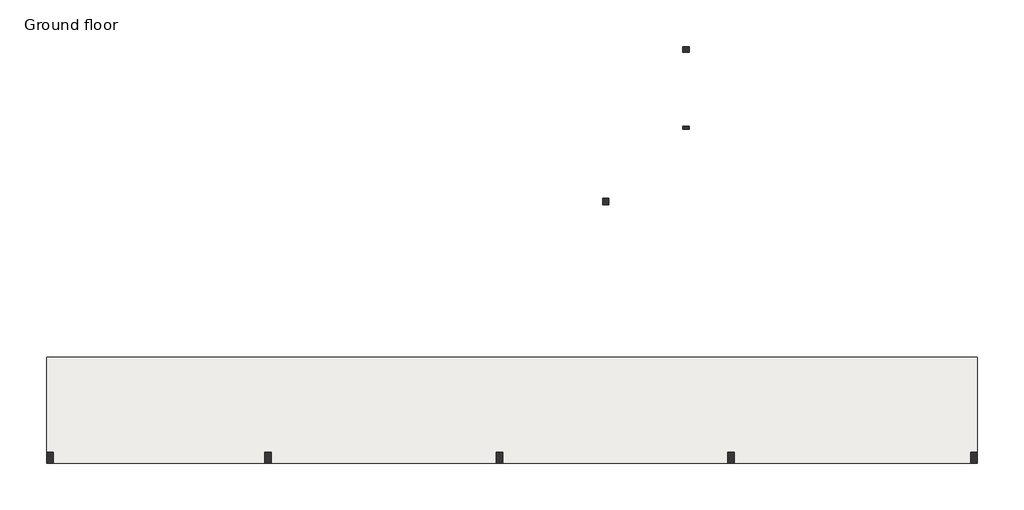
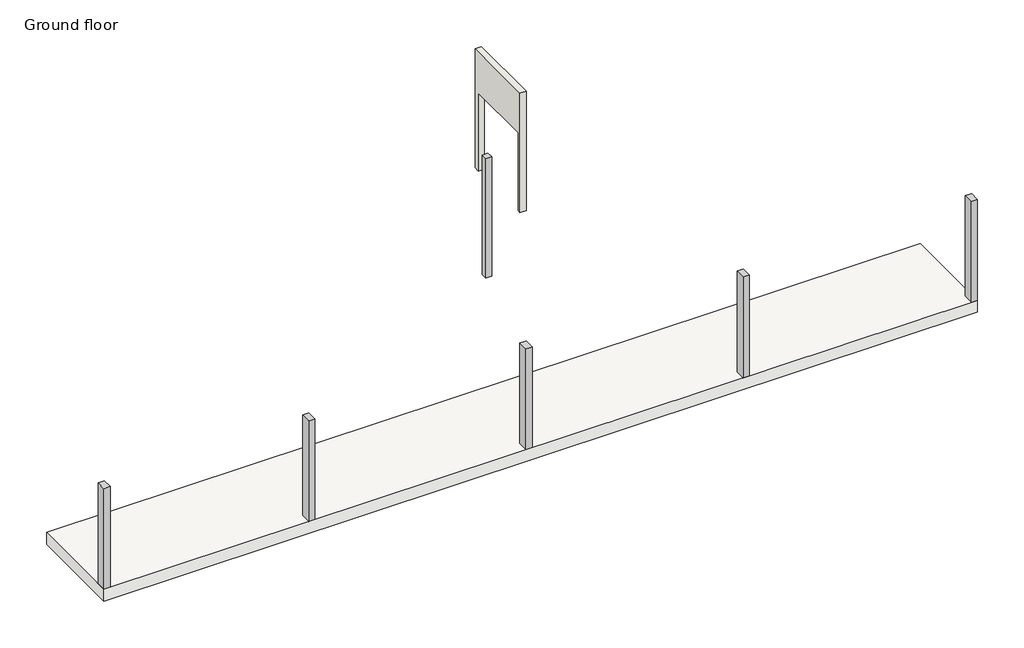
# One storey: 6 columns, 1 slab, 1 wall.
"""IFC4 building model written with IfcOpenShell, lengths in millimetres."""

import ifcopenshell
import ifcopenshell.guid

model = None  # the IFC model being written
_history = None  # IfcOwnerHistory: only IFC2X3 demands one
_inside = {}  # id of a spatial element -> (the spatial element, [elements in it])
_under = {}  # id of a project, library or spatial element -> (it, [spatial elements below it])
_declared = {}  # id of a project -> (the project, [libraries it declares])
_typed = {}  # id of a type object -> (the type object, [elements of that type])
_made_of = {}  # id of a material, layer set ... -> (it, [elements and type objects made of it])


def new_model(schema):
    """Start an empty IFC model of exactly this schema.

    Asked for "IFC4X3", IfcOpenShell would pick the latest addendum, in which some entities
    have other attributes; the version numbers below select the first issue.
    IFC2X3 requires an IfcOwnerHistory on every rooted entity: one is made here for all.
    """
    global model, _history
    if schema == "IFC4X3":
        model = ifcopenshell.file(schema_version=(4, 3, 0, 0))
    else:
        model = ifcopenshell.file(schema=schema)
    _inside.clear()
    _under.clear()
    _declared.clear()
    _typed.clear()
    _made_of.clear()
    _history = None
    if model.schema == "IFC2X3":
        org = make("IfcOrganization", Name="unknown")
        user = make(
            "IfcPersonAndOrganization",
            ThePerson=make("IfcPerson", FamilyName="unknown"),
            TheOrganization=org,
        )
        app = make(
            "IfcApplication",
            ApplicationDeveloper=org,
            Version="unknown",
            ApplicationFullName="unknown",
            ApplicationIdentifier="unknown",
        )
        _history = make(
            "IfcOwnerHistory",
            OwningUser=user,
            OwningApplication=app,
            ChangeAction="ADDED",
            CreationDate=0,
        )
    return model


def make(cls, **values):
    """One entity of the class cls with the attributes given. An attribute that is None is left unset."""
    return model.create_entity(
        cls, **{name: value for name, value in values.items() if value is not None}
    )


def rooted(cls, **values):
    """An entity with a GlobalId (a new one), such as an element, a storey or a relation."""
    return make(cls, GlobalId=ifcopenshell.guid.new(), OwnerHistory=_history, **values)


def si_unit(unit_type, name, prefix=None):
    """IfcSIUnit, for example si_unit("LENGTHUNIT", "METRE", prefix="MILLI")."""
    return make("IfcSIUnit", UnitType=unit_type, Prefix=prefix, Name=name)


def assignment(units):
    """IfcUnitAssignment: the units of a project."""
    return None if units is None else make("IfcUnitAssignment", Units=units)


def point(xyz):
    """IfcCartesianPoint."""
    return None if xyz is None else make("IfcCartesianPoint", Coordinates=xyz)


def direction(xyz):
    """IfcDirection."""
    return None if xyz is None else make("IfcDirection", DirectionRatios=xyz)


def frame(location, z_axis=None, x_axis=None):
    """IfcAxis2Placement3D, a coordinate frame: its origin and axes. An axis left out is left unset."""
    return make(
        "IfcAxis2Placement3D",
        Location=point(location),
        Axis=direction(z_axis),
        RefDirection=direction(x_axis),
    )


def origin():
    """The frame at (0, 0, 0) with its axes left unset."""
    return frame((0.0, 0.0, 0.0))


def origin_with_axes():
    """The frame at (0, 0, 0) with the z axis (0, 0, 1) and the x axis (1, 0, 0) written out."""
    return frame((0.0, 0.0, 0.0), z_axis=(0.0, 0.0, 1.0), x_axis=(1.0, 0.0, 0.0))


def place(relative_to, where):
    """IfcLocalPlacement: puts the frame where relative to a parent placement (None: the world)."""
    return make(
        "IfcLocalPlacement", PlacementRelTo=relative_to, RelativePlacement=where
    )


def context(
    kind, dimensions, precision=None, world=None, true_north=None, identifier=None
):
    """IfcGeometricRepresentationContext, for example the 3D "Model" context."""
    return make(
        "IfcGeometricRepresentationContext",
        ContextIdentifier=identifier,
        ContextType=kind,
        CoordinateSpaceDimension=dimensions,
        Precision=precision,
        WorldCoordinateSystem=world,
        TrueNorth=true_north,
    )


def project(units=None, contexts=None):
    """IfcProject with its units and contexts."""
    return rooted(
        "IfcProject",
        Name="project",
        RepresentationContexts=contexts,
        UnitsInContext=assignment(units),
    )


def spatial(cls, under=None, at=None, **own):
    """A site, building, storey or space (cls), placed at a placement, below another one or the project."""
    s = rooted(cls, ObjectPlacement=at, **own)
    if under is not None:
        _under.setdefault(under.id(), (under, []))[1].append(s)
    return s


def polyline(points):
    """IfcPolyline through the points."""
    return make("IfcPolyline", Points=[point(p) for p in points])


def outline(outer, holes=None, kind="AREA"):
    """IfcArbitraryClosedProfileDef: a profile drawn as a closed curve; with holes, ...WithVoids."""
    if holes is None:
        return make("IfcArbitraryClosedProfileDef", ProfileType=kind, OuterCurve=outer)
    return make(
        "IfcArbitraryProfileDefWithVoids",
        ProfileType=kind,
        OuterCurve=outer,
        InnerCurves=holes,
    )


def extrude(swept, where, along, depth):
    """IfcExtrudedAreaSolid: the profile swept, set in the frame where, extruded along a direction by depth."""
    return make(
        "IfcExtrudedAreaSolid",
        SweptArea=swept,
        Position=where,
        ExtrudedDirection=direction(along),
        Depth=depth,
    )


def shape(context_of_items, identifier, shape_type, items):
    """IfcShapeRepresentation: the items that make up one representation, for example the "Body"."""
    return make(
        "IfcShapeRepresentation",
        ContextOfItems=context_of_items,
        RepresentationIdentifier=identifier,
        RepresentationType=shape_type,
        Items=items,
    )


def source(mapping_origin, context_of_items, identifier, shape_type, items):
    """IfcRepresentationMap: a shape defined once, which mapped items show again and again."""
    return make(
        "IfcRepresentationMap",
        MappingOrigin=mapping_origin,
        MappedRepresentation=shape(context_of_items, identifier, shape_type, items),
    )


def transform(
    local_origin,
    x_axis=None,
    y_axis=None,
    z_axis=None,
    scale=None,
    scale2=None,
    scale3=None,
    uniform=True,
):
    """IfcCartesianTransformationOperator3D, or its non-uniform kind. x_axis, y_axis, z_axis: its Axis1, 2, 3."""
    if uniform:
        return make(
            "IfcCartesianTransformationOperator3D",
            Axis1=direction(x_axis),
            Axis2=direction(y_axis),
            LocalOrigin=point(local_origin),
            Scale=scale,
            Axis3=direction(z_axis),
        )
    return make(
        "IfcCartesianTransformationOperator3DnonUniform",
        Axis1=direction(x_axis),
        Axis2=direction(y_axis),
        LocalOrigin=point(local_origin),
        Scale=scale,
        Axis3=direction(z_axis),
        Scale2=scale2,
        Scale3=scale3,
    )


def mapped(mapping_source, mapping_target):
    """IfcMappedItem: shows the shape of a source again, moved by a transform."""
    return make(
        "IfcMappedItem", MappingSource=mapping_source, MappingTarget=mapping_target
    )


def made_of(thing, what):
    """Note that an element or type object is made of a material, layer set ...; save() writes the relation."""
    if what is not None:
        _made_of.setdefault(what.id(), (what, []))[1].append(thing)
    return thing


def element(
    cls,
    number,
    at=None,
    inside=None,
    cuts=None,
    type_object=None,
    material=None,
    context=None,
    identifier="Body",
    shape_type=None,
    held_by="IfcProductDefinitionShape",
    body=None,
    shapes=None,
    **own,
):
    """One element of the class cls, such as IfcWall. Its Tag is "e" and its number.

    at: its placement. inside: the storey or other place that contains it. cuts: it is an
    opening in that element (IfcRelVoidsElement). A single representation is given by context,
    identifier, shape_type and body (its items); several are given by shapes. held_by: the class
    of the entity that holds the representations. save() writes the other relations.
    """
    e = rooted(cls, Tag="e%d" % number, ObjectPlacement=at, **own)
    if body is not None:
        shapes = [shape(context, identifier, shape_type, body)]
    if shapes is not None:
        e.Representation = make(held_by, Representations=shapes)
    if inside is not None:
        _inside.setdefault(inside.id(), (inside, []))[1].append(e)
    if cuts is not None:
        rooted(
            "IfcRelVoidsElement", RelatingBuildingElement=cuts, RelatedOpeningElement=e
        )
    if type_object is not None:
        _typed.setdefault(type_object.id(), (type_object, []))[1].append(e)
    return made_of(e, material)


def aggregate(whole, parts):
    """IfcRelAggregates: a whole, such as a stair, and the parts it consists of."""
    return rooted("IfcRelAggregates", RelatingObject=whole, RelatedObjects=parts)


def save(model, path):
    """Write the relations noted so far, then the file.

    IfcRelAggregates (storeys below a building ...), IfcRelContainedInSpatialStructure (elements
    in a storey), IfcRelDefinesByType, IfcRelAssociatesMaterial and IfcRelDeclares: one each for
    every whole, place, type object, material and project.
    """
    for whole, parts in _under.values():
        aggregate(whole, parts)
    for where, things in _inside.values():
        rooted(
            "IfcRelContainedInSpatialStructure",
            RelatedElements=things,
            RelatingStructure=where,
        )
    for kind, things in _typed.values():
        rooted("IfcRelDefinesByType", RelatedObjects=things, RelatingType=kind)
    for what, things in _made_of.values():
        rooted("IfcRelAssociatesMaterial", RelatedObjects=things, RelatingMaterial=what)
    for by, libraries in _declared.values():
        rooted("IfcRelDeclares", RelatingContext=by, RelatedDefinitions=libraries)
    model.write(path)


def column_1c9a027e(model_context):
    return source(origin(), model_context, "Body", "SweptSolid", [
        extrude(outline(polyline([(76.2, 127.0), (76.2, -127.0), (-76.2, -127.0), (-76.2, 127.0), (76.2, 127.0)])), origin_with_axes(), (0.0, 0.0, 1.0), 2628.9),
    ])


def timber_column_6x5_2_9af8efbf(model_context):
    return source(origin(), model_context, "Body", "SweptSolid", [
        extrude(outline(polyline([(69.85, 76.2), (69.85, -76.2), (-69.85, -76.2), (-69.85, 76.2), (69.85, 76.2)])), origin_with_axes(), (0.0, 0.0, 1.0), 3111.5),
    ])


model = new_model("IFC4")

# Units and contexts
model_context = context("Model", 3, world=origin())
ifc_project = project(units=[si_unit("LENGTHUNIT", "METRE", prefix="MILLI")], contexts=[model_context])

# Site, building, storey
site = spatial("IfcSite", under=ifc_project)
building = spatial("IfcBuilding", under=site)
storey = spatial("IfcBuildingStorey", under=building, Name="Ground floor", Elevation=0.0)

# Columns
placement = place(None, origin())
column_shape = column_1c9a027e(model_context)
element("IfcColumn", 1, ObjectType="Timber-Column : 10\" x 6\"", at=placement, inside=storey, context=model_context, shape_type="MappedRepresentation", body=[
    mapped(column_shape, transform((7576.3370052, 318.7615366, 0.0), x_axis=(1.0, 0.0, 0.0), y_axis=(0.0, 1.0, 0.0), z_axis=(0.0, 0.0, 1.0))),
])
element("IfcColumn", 2, ObjectType="Timber-Column : 10\" x 6\"", at=placement, inside=storey, context=model_context, shape_type="MappedRepresentation", body=[
    mapped(column_shape, transform((28956.7870052, 318.7615366, 0.0), x_axis=(1.0, 0.0, 0.0), y_axis=(0.0, 1.0, 0.0), z_axis=(0.0, 0.0, 1.0))),
])
element("IfcColumn", 3, ObjectType="Timber-Column : 10\" x 6\"", at=placement, inside=storey, context=model_context, shape_type="MappedRepresentation", body=[
    mapped(column_shape, transform((23330.6870052, 318.7615366, 0.0), x_axis=(1.0, 0.0, 0.0), y_axis=(0.0, 1.0, 0.0), z_axis=(0.0, 0.0, 1.0))),
])
element("IfcColumn", 4, ObjectType="Timber-Column : 10\" x 6\"", at=placement, inside=storey, context=model_context, shape_type="MappedRepresentation", body=[
    mapped(column_shape, transform((17977.6370052, 318.7615366, 0.0), x_axis=(1.0, 0.0, 0.0), y_axis=(0.0, 1.0, 0.0), z_axis=(0.0, 0.0, 1.0))),
])
element("IfcColumn", 5, ObjectType="Timber-Column : 10\" x 6\"", at=placement, inside=storey, context=model_context, shape_type="MappedRepresentation", body=[
    mapped(column_shape, transform((12624.5870052, 318.7615366, 0.0), x_axis=(1.0, 0.0, 0.0), y_axis=(0.0, 1.0, 0.0), z_axis=(0.0, 0.0, 1.0))),
])
timber_column_6x5_2_shape = timber_column_6x5_2_9af8efbf(model_context)
element("IfcColumn", 6, ObjectType="Timber-Column : 6x5 2", at=placement, inside=storey, context=model_context, shape_type="MappedRepresentation", body=[
    mapped(timber_column_6x5_2_shape, transform((20435.0870052, 6243.3115366, 0.0), x_axis=(1.0, 0.0, 0.0), y_axis=(0.0, 1.0, 0.0), z_axis=(0.0, 0.0, 1.0))),
])

# Slab
element("IfcSlab", 7, ObjectType="Generic - 12\"", at=placement, inside=storey, context=model_context, shape_type="SweptSolid", body=[
    extrude(outline(polyline([(7500.1370052, 191.7615366), (7500.1370052, 2642.8615366), (29032.9870052, 2642.8615366), (29032.9870052, 191.7615366), (7500.1370052, 191.7615366)])), frame((0.0, 0.0, -304.8), z_axis=(0.0, 0.0, 1.0), x_axis=(1.0, 0.0, 0.0)), (0.0, 0.0, 1.0), 304.8),
])

# Wall
element("IfcWall", 8, ObjectType="Generic - 6\"", at=placement, inside=storey, context=model_context, shape_type="SweptSolid", body=[
    extrude(outline(polyline([(7989.5615366, 2032.0), (7989.5615366, 0.0), (7913.3615366, 0.0), (7913.3615366, 3111.5), (9831.0615366, 3111.5), (9831.0615366, 0.0), (9697.7115366, 0.0), (9697.7115366, 2032.0), (7989.5615366, 2032.0)])), frame((22213.0870052, 0.0, 0.0), z_axis=(1.0, 0.0, 0.0), x_axis=(0.0, 1.0, 0.0)), (0.0, 0.0, 1.0), 152.4),
])

save(model, "model.ifc")

# Revit data of these elements
# Type "Timber-Column : 10\" x 6\""
#   Assembly Code = "B10"
#   A = 0.140625 SF
#   b = 0' - 6"
#   d = 0' - 10"
#   Structural Material [instance default] = Softwood, Lumber
# Type "Timber-Column : 6x5 2"
#   Assembly Code = "B10"
#   A = 0.140625 SF
#   b = 0' - 5 1/2"
#   d = 0' - 6"
#   Structural Material [instance default] = Softwood, Lumber
# Type "Generic - 12\""
#   Assembly Code = "B1010"
#   Function = 0
#   Layers, outside or top first: 1' - 0" no material (function 1)
# Type "Generic - 6\""
#   Assembly Code = "B2010"
#   Layers, outside or top first: 0' - 6" no material (function 1)
# Elements 1, 2, 3, 4, 5 (IfcColumn, "Timber-Column : 10\" x 6\"")
#   Structural Material = Softwood, Lumber
#   Phase Created = New Construction
#   Materials on its faces: "Softwood, Lumber"
# Element 6 (IfcColumn, "Timber-Column : 6x5 2")
#   Structural Material = Softwood, Lumber
#   Phase Created = New Construction
#   Materials on its faces: "Softwood, Lumber"
# Element 7 (IfcSlab, "Generic - 12\"")
#   built-in parameter 1001955 = -1.5708 (stored number, unit not read)
#   Height Offset From Level = 0' - 0"
#   Phase Created = New Construction
#   Materials on its faces: "Default Floor"
# Element 8 (IfcWall, "Generic - 6\"")
#   Top Offset = 0' - 0"
#   Base Offset = 0' - 0"
#   wall height = 10' - 2 1/2"
#   Phase Created = New Construction
#   Base Constraint = Ground floor
#   Top Constraint = Top of walls
#   Materials on its faces: "Default Wall"
# Materials
#   "Softwood, Lumber": class "Wood", colour RGB 144 113 62, transparency 0, Description = "Pinus Echinata", Cost = 0
#   "Default Floor": class "Miscellaneous", colour RGB 80 80 80, transparency 0
#   "Default Wall": class "Miscellaneous", colour RGB 80 80 80, transparency 0
